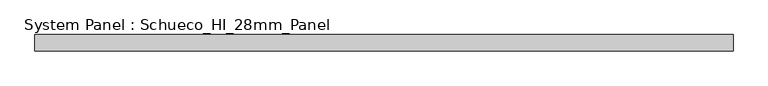
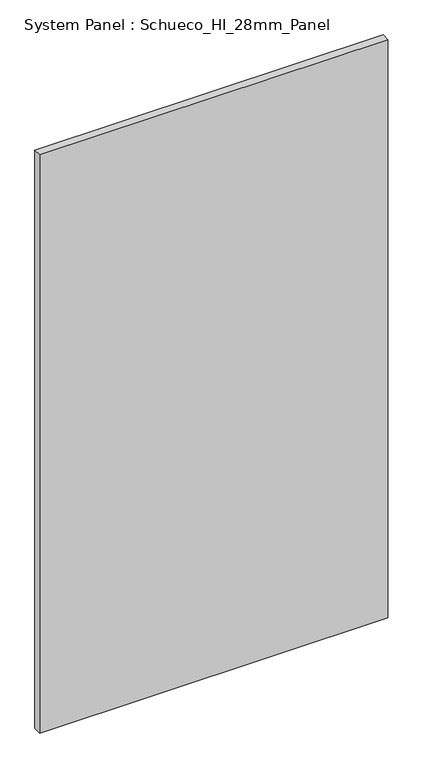
"""IFC4 building model written with IfcOpenShell, lengths in millimetres: plate geometry, System Panel : Schueco_HI_28mm_Panel."""

from ifc_helpers import new_model, si_unit, origin, origin_with_axes, place, context, project, spatial, polyline, outline, extrude, source, transform, mapped, element, save


def system_panel_schueco_hi_28mm_panel_cfb62f5e(model_context):
    return source(origin(), model_context, "Body", "SweptSolid", [
        extrude(outline(polyline([(606.5, -28.0), (-606.5, -28.0), (-606.5, 0.0), (606.5, 0.0), (606.5, -28.0)])), origin_with_axes(), (0.0, 0.0, 1.0), 2128.0),
    ])


if __name__ == "__main__":
    model = new_model("IFC4")
    model_context = context("Model", 3, world=origin())
    ifc_project = project(units=[si_unit("LENGTHUNIT", "METRE", prefix="MILLI")], contexts=[model_context])
    site = spatial("IfcSite", under=ifc_project)
    building = spatial("IfcBuilding", under=site)
    placement = place(None, origin())
    system_panel_schueco_hi_28mm_panel_shape = system_panel_schueco_hi_28mm_panel_cfb62f5e(model_context)
    element("IfcPlate", 1, ObjectType="System Panel : Schueco_HI_28mm_Panel", at=placement, inside=building, context=model_context, shape_type="MappedRepresentation", body=[
        mapped(system_panel_schueco_hi_28mm_panel_shape, transform((0.0, 0.0, 0.0), x_axis=(1.0, 0.0, 0.0), y_axis=(0.0, 1.0, 0.0), z_axis=(0.0, 0.0, 1.0))),
    ])
    save(model, "model.ifc")

# Revit data of these elements
# Type "System Panel : Schueco_HI_28mm_Panel"
#   Model = "Panel 28mm"
# Element 1 (IfcPlate, "System Panel : Schueco_HI_28mm_Panel")
#   Materials on its faces: "Alu"
# Materials
#   "Alu": class "Glas", colour RGB 140 140 140, transparency 0
